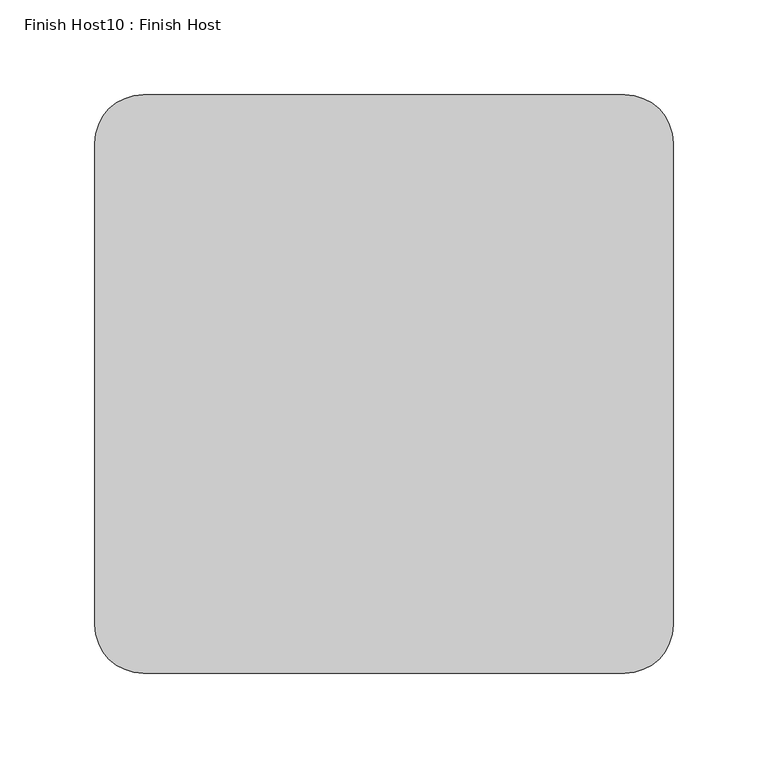
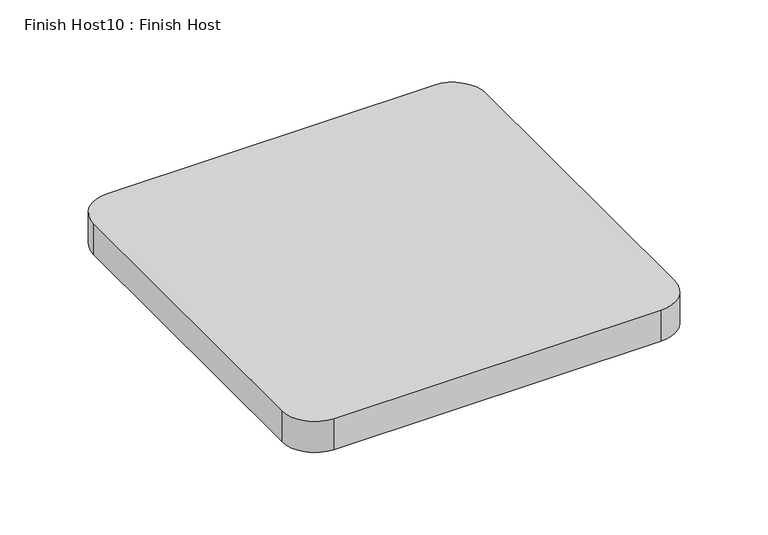
"""IFC4 building model written with IfcOpenShell, lengths in millimetres: proxy geometry, Finish Host10 : Finish Host."""

from ifc_helpers import new_model, si_unit, point, frame_2d, origin, origin_with_axes, place, context, project, spatial, polyline, circle_curve, trimmed, segment, composite_curve, outline, extrude, source, transform, mapped, element, save


def finish_host10_finish_host_44f99bfc(model_context):
    return source(origin(), model_context, "Body", "SweptSolid", [
        extrude(outline(composite_curve([segment(polyline([(701.4157184, 3462.3960864), (701.4157184, 3716.3960864)]), True, "CONTINUOUS"), segment(trimmed(circle_curve(frame_2d((726.8157184, 3716.3960864)), 25.4), [point((701.4157184, 3716.3960864))], [point((726.8157184, 3741.7960864))], False, "CARTESIAN"), True, "CONTINUOUS"), segment(polyline([(726.8157184, 3741.7960864), (980.8157184, 3741.7960864)]), True, "CONTINUOUS"), segment(trimmed(circle_curve(frame_2d((980.8157184, 3716.3960864)), 25.4), [point((980.8157184, 3741.7960864))], [point((1006.2157184, 3716.3960864))], False, "CARTESIAN"), True, "CONTINUOUS"), segment(polyline([(1006.2157184, 3716.3960864), (1006.2157184, 3462.3960864)]), True, "CONTINUOUS"), segment(trimmed(circle_curve(frame_2d((980.8157184, 3462.3960864)), 25.4), [point((1006.2157184, 3462.3960864))], [point((980.8157184, 3436.9960864))], False, "CARTESIAN"), True, "CONTINUOUS"), segment(polyline([(980.8157184, 3436.9960864), (726.8157184, 3436.9960864)]), True, "CONTINUOUS"), segment(trimmed(circle_curve(frame_2d((726.8157184, 3462.3960864)), 25.4), [point((726.8157184, 3436.9960864))], [point((701.4157184, 3462.3960864))], False, "CARTESIAN"), True, "CONTINUOUS")], self_intersect=False)), origin_with_axes(), (0.0, 0.0, 1.0), 25.4),
    ])


if __name__ == "__main__":
    model = new_model("IFC4")
    model_context = context("Model", 3, world=origin())
    ifc_project = project(units=[si_unit("LENGTHUNIT", "METRE", prefix="MILLI")], contexts=[model_context])
    site = spatial("IfcSite", under=ifc_project)
    building = spatial("IfcBuilding", under=site)
    placement = place(None, origin())
    finish_host10_finish_host_shape = finish_host10_finish_host_44f99bfc(model_context)
    element("IfcBuildingElementProxy", 1, Name="Finish Host10 : Finish Host", ObjectType="Finish Host10 : Finish Host", at=placement, inside=building, context=model_context, shape_type="MappedRepresentation", body=[
        mapped(finish_host10_finish_host_shape, transform((0.0, 0.0, 0.0), x_axis=(1.0, 0.0, 0.0), y_axis=(0.0, 1.0, 0.0), z_axis=(0.0, 0.0, 1.0))),
    ])
    save(model, "model.ifc")

# Revit data of these elements
# Type "Finish Host10 : Finish Host"
#   Countertop Material = Fabric - Teknion - S142 - Synaptic - Transmission
# Element 1 (IfcBuildingElementProxy, "Finish Host10 : Finish Host")
#   Materials on its faces: "Fabric - Teknion - S142 - Synaptic - Transmission"
# Materials
#   "Fabric - Teknion - S142 - Synaptic - Transmission": class "Fabric", colour RGB 22 25 28, transparency 0, Model = "S142", Manufacturer = "Teknion Studio", URL = "http://www.teknionstudio.com/", Description = "Transmission Synaptic", Cost = 0
